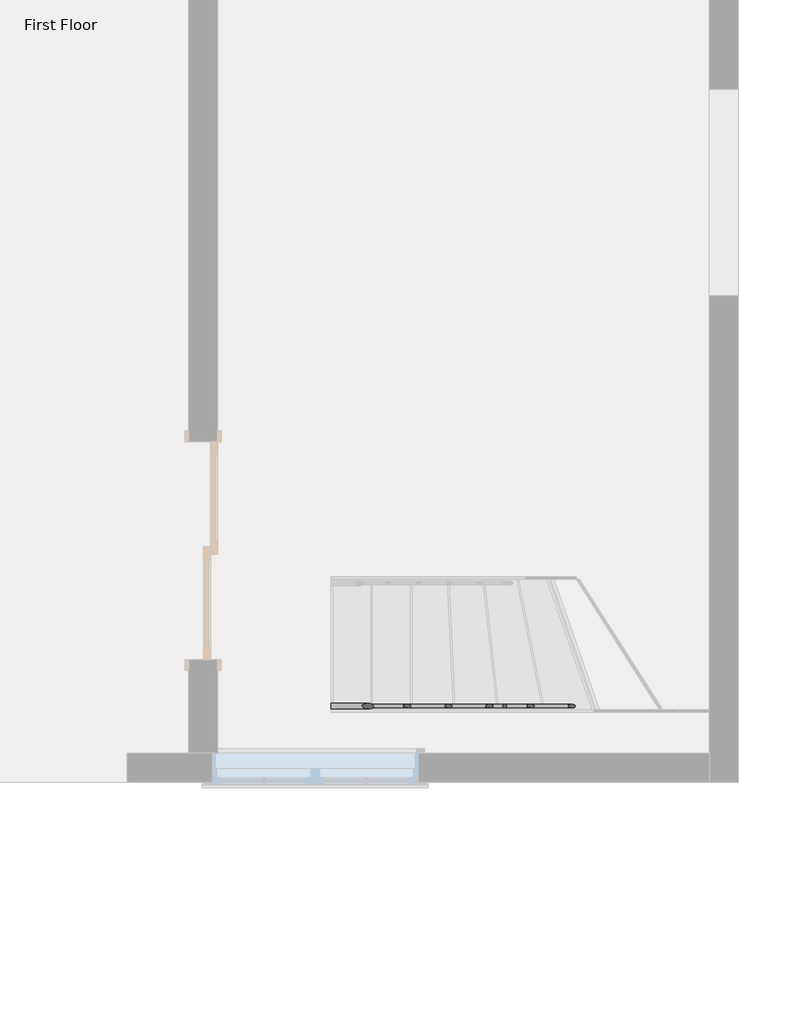
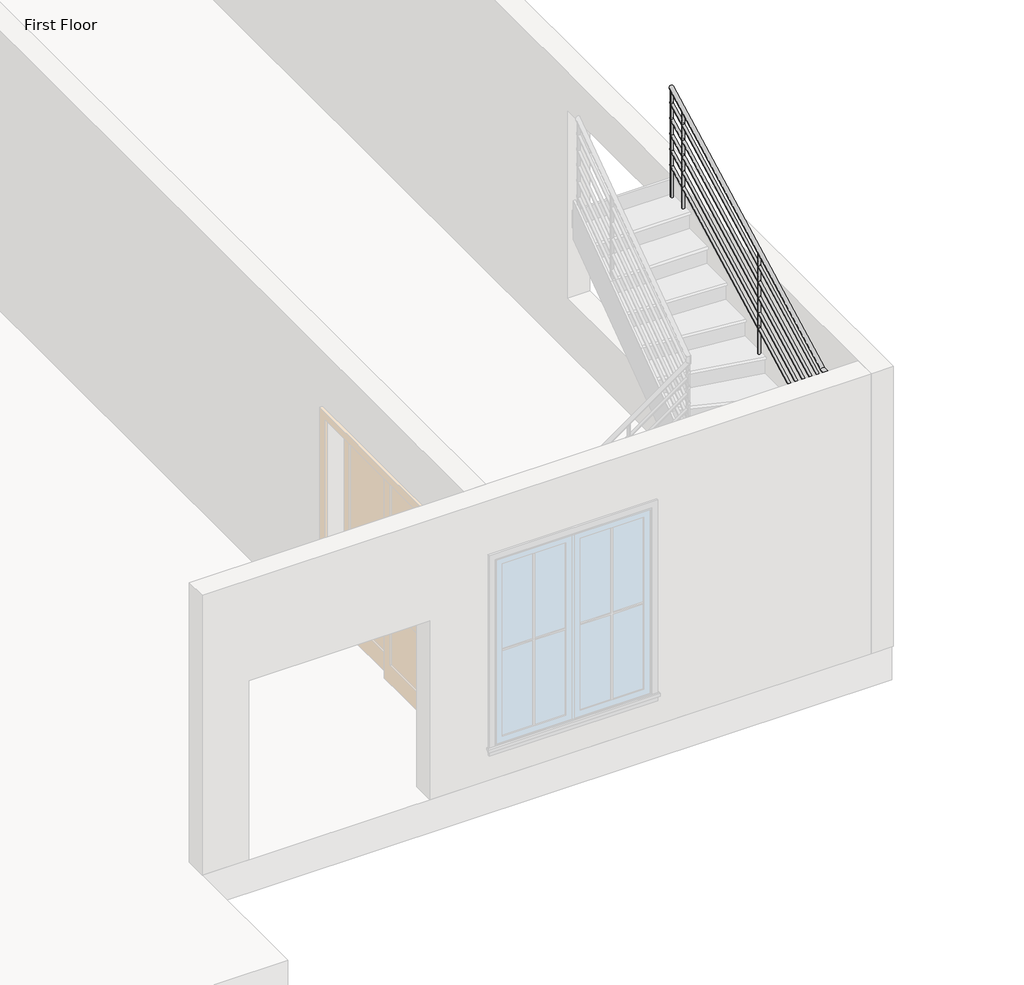
# One storey, part 3 of 4: 1 railing.
"""IFC4 building model written with IfcOpenShell, lengths in millimetres."""

from ifc_helpers import new_model, si_unit, point, frame, frame_2d, origin, place, context, project, spatial, circle_curve, ellipse_curve, trimmed, segment, composite_curve, outline, extrude, element, save
from ifc_brep_helpers import plane_surface, cylinder_surface, advanced_brep

model = new_model("IFC4")

# Units and contexts
model_context = context("Model", 3, world=origin())
ifc_project = project(units=[si_unit("LENGTHUNIT", "METRE", prefix="MILLI")], contexts=[model_context])

# Site, building, storey
site = spatial("IfcSite", under=ifc_project)
building = spatial("IfcBuilding", under=site)
storey = spatial("IfcBuildingStorey", under=building, Name="First Floor", Elevation=0.0)

# Railing
placement = place(None, origin())
element("IfcRailing", 1, ObjectType="Handrail - Pipe", at=placement, inside=storey, context=model_context, shape_type="SolidModel", body=[
    advanced_brep(
    [(6778.2616192, -13382.7029211, 1064.3134281), (6778.2616192, -13344.6029211, 1064.3134281), (9221.3605111, -13382.7029211, 2352.675), (9221.3605111, -13344.6029211, 2352.675), (9390.3486087, -13344.6029211, 2352.675), (9428.4486087, -13382.7029211, 2352.675), (9428.4486087, -13166.1843326, 2352.675), (9390.3486087, -13166.1843326, 2352.675), (9428.4486087, -10732.5159316, 3636.0634281), (9390.3486087, -10732.5159316, 3636.0634281)],
    [
        (0, 1, ellipse_curve(frame((6778.2616192, -13363.6529211, 1064.3134281), z_axis=(-1.0, 0.0, 0.0), x_axis=(0.0, 0.0, -1.0)), 21.5365719, 19.05)),
        (1, 0, ellipse_curve(frame((6778.2616192, -13363.6529211, 1064.3134281), z_axis=(-1.0, 0.0, 0.0), x_axis=(0.0, 0.0, -1.0)), 21.5365719, 19.05)),
        (0, 2),
        (2, 3, ellipse_curve(frame((9221.3605111, -13363.6529211, 2352.675), z_axis=(-0.9707064153254982, 0.0, -0.24026871466323146), x_axis=(0.2402687146632313, 0.0, -0.9707064153254984)), 19.6248832, 19.05)),
        (3, 1),
        (3, 2, ellipse_curve(frame((9221.3605111, -13363.6529211, 2352.675), z_axis=(-0.9707064153254982, 0.0, -0.24026871466323146), x_axis=(0.2402687146632313, 0.0, -0.9707064153254984)), 19.6248832, 19.05)),
        (4, 5, ellipse_curve(frame((9409.3986087, -13363.6529211, 2352.675), z_axis=(0.7071067811865475, 0.7071067811865475, 0.0), x_axis=(0.7071067811865474, -0.7071067811865476, 0.0)), 26.9407684, 19.05)),
        (5, 6),
        (6, 7, ellipse_curve(frame((9409.3986087, -13166.1843326, 2352.675), z_axis=(0.0, -0.9707064153254983, -0.2402687146632317), x_axis=(0.0, -0.24026871466323058, 0.9707064153254984)), 19.6248832, 19.05)),
        (7, 4),
        (5, 4, ellipse_curve(frame((9409.3986087, -13363.6529211, 2352.675), z_axis=(0.7071067811865475, 0.7071067811865475, 0.0), x_axis=(0.7071067811865474, -0.7071067811865476, 0.0)), 26.9407684, 19.05)),
        (7, 6, ellipse_curve(frame((9409.3986087, -13166.1843326, 2352.675), z_axis=(0.0, -0.9707064153254983, -0.2402687146632317), x_axis=(0.0, -0.24026871466323058, 0.9707064153254984)), 19.6248832, 19.05)),
        (2, 5),
        (4, 3),
        (8, 9, ellipse_curve(frame((9409.3986087, -10732.5159316, 3636.0634281), z_axis=(0.0, 1.0, 0.0), x_axis=(0.0, 0.0, -1.0)), 21.5365719, 19.05)),
        (9, 8, ellipse_curve(frame((9409.3986087, -10732.5159316, 3636.0634281), z_axis=(0.0, 1.0, 0.0), x_axis=(0.0, 0.0, -1.0)), 21.5365719, 19.05)),
        (6, 8),
        (9, 7),
    ],
    [
        plane_surface(frame((6778.2616192, -13363.6529211, 1085.85), z_axis=(-1.0, 0.0, 0.0), x_axis=(0.0, 1.0, 0.0))),
        cylinder_surface(frame((6787.1476968, -13363.6529211, 1068.999477), z_axis=(-0.8845418895081573, 0.0, -0.4664607654512208), x_axis=(0.0, 1.0, 0.0)), 19.05),
        cylinder_surface(frame((9409.3986087, -13363.6529211, 2352.675), z_axis=(0.0, -1.0, 0.0), x_axis=(-1.0, 0.0, 0.0)), 19.05),
        cylinder_surface(frame((9216.6452657, -13363.6529211, 2352.675), z_axis=(-1.0, 0.0, 0.0), x_axis=(0.0, 1.0, 0.0)), 19.05),
        plane_surface(frame((9409.3986087, -10732.5159316, 3657.6), z_axis=(0.0, 1.0, 0.0), x_axis=(0.0, 0.0, 1.0))),
        cylinder_surface(frame((9409.3986087, -13162.0135005, 2354.874477), z_axis=(0.0, -0.8845418895081572, -0.4664607654512212), x_axis=(-1.0, 0.0, 0.0)), 19.05),
    ],
    [
        (0, [[1, 2]]),
        (1, [[-1, 3, 4, 5]]),
        (1, [[-2, -5, 6, -3]]),
        (2, [[7, 8, 9, 10]]),
        (2, [[11, -10, 12, -8]]),
        (3, [[-4, 13, -7, 14]]),
        (3, [[-6, -14, -11, -13]]),
        (4, [[15, 16]]),
        (5, [[-9, 17, -16, 18]]),
        (5, [[-12, -18, -15, -17]]),
    ],
),
    advanced_brep(
    [(6778.2616192, -13350.9529211, 919.0922854), (6778.2616192, -13376.3529211, 919.0922854), (9219.7887626, -13350.9529211, 2206.625), (9219.7887626, -13376.3529211, 2206.625), (9396.6986087, -13350.9529211, 2206.625), (9396.6986087, -13376.3529211, 2206.625)],
    [
        (0, 1, ellipse_curve(frame((6778.2616192, -13363.6529211, 919.0922854), z_axis=(-1.0, 0.0, 0.0), x_axis=(0.0, 0.0, -1.0)), 14.3577146, 12.7)),
        (1, 0, ellipse_curve(frame((6778.2616192, -13363.6529211, 919.0922854), z_axis=(-1.0, 0.0, 0.0), x_axis=(0.0, 0.0, -1.0)), 14.3577146, 12.7)),
        (0, 2),
        (2, 3, ellipse_curve(frame((9219.7887626, -13363.6529211, 2206.625), z_axis=(-0.9707064153254982, 0.0, -0.24026871466323146), x_axis=(0.2402687146632313, 0.0, -0.9707064153254984)), 13.0832555, 12.7)),
        (3, 1),
        (3, 2, ellipse_curve(frame((9219.7887626, -13363.6529211, 2206.625), z_axis=(-0.9707064153254982, 0.0, -0.24026871466323146), x_axis=(0.2402687146632313, 0.0, -0.9707064153254984)), 13.0832555, 12.7)),
        (4, 5, circle_curve(frame((9396.6986087, -13363.6529211, 2206.625), z_axis=(1.0, 0.0, 0.0), x_axis=(0.0, -1.0, 0.0)), 12.7)),
        (5, 4, circle_curve(frame((9396.6986087, -13363.6529211, 2206.625), z_axis=(1.0, 0.0, 0.0), x_axis=(0.0, -1.0, 0.0)), 12.7)),
        (2, 4),
        (5, 3),
    ],
    [
        plane_surface(frame((6778.2616192, -13363.6529211, 933.45), z_axis=(-1.0, 0.0, 0.0), x_axis=(0.0, 1.0, 0.0))),
        cylinder_surface(frame((6784.185671, -13363.6529211, 922.216318), z_axis=(-0.8845418895081573, 0.0, -0.4664607654512208), x_axis=(0.0, -1.0, 0.0)), 12.7),
        plane_surface(frame((9396.6986087, -13363.6529211, 2219.325), z_axis=(1.0, 0.0, 0.0), x_axis=(0.0, 1.0, 0.0))),
        cylinder_surface(frame((9216.6452657, -13363.6529211, 2206.625), z_axis=(-1.0, 0.0, 0.0), x_axis=(0.0, -1.0, 0.0)), 12.7),
    ],
    [
        (0, [[1, 2]]),
        (1, [[-1, 3, 4, 5]]),
        (1, [[-2, -5, 6, -3]]),
        (2, [[7, 8]]),
        (3, [[-4, 9, -8, 10]]),
        (3, [[-6, -10, -7, -9]]),
    ],
),
    advanced_brep(
    [(9396.6986087, -13376.3529211, 2206.625), (9422.0986087, -13376.3529211, 2206.625), (9396.6986087, -13167.7560811, 2206.625), (9422.0986087, -13167.7560811, 2206.625), (9396.6986087, -10732.5159316, 3490.8422854), (9422.0986087, -10732.5159316, 3490.8422854)],
    [
        (0, 1, circle_curve(frame((9409.3986087, -13376.3529211, 2206.625), z_axis=(0.0, -1.0, 0.0), x_axis=(1.0, 0.0, 0.0)), 12.7)),
        (1, 0, circle_curve(frame((9409.3986087, -13376.3529211, 2206.625), z_axis=(0.0, -1.0, 0.0), x_axis=(1.0, 0.0, 0.0)), 12.7)),
        (0, 2),
        (2, 3, ellipse_curve(frame((9409.3986087, -13167.7560811, 2206.625), z_axis=(0.0, -0.9707064153254982, -0.24026871466323177), x_axis=(0.0, -0.2402687146632315, 0.9707064153254982)), 13.0832555, 12.7)),
        (3, 1),
        (3, 2, ellipse_curve(frame((9409.3986087, -13167.7560811, 2206.625), z_axis=(0.0, -0.9707064153254982, -0.24026871466323177), x_axis=(0.0, -0.2402687146632315, 0.9707064153254982)), 13.0832555, 12.7)),
        (4, 5, ellipse_curve(frame((9409.3986087, -10732.5159316, 3490.8422854), z_axis=(0.0, 1.0, 0.0), x_axis=(0.0, 0.0, -1.0)), 14.3577146, 12.7)),
        (5, 4, ellipse_curve(frame((9409.3986087, -10732.5159316, 3490.8422854), z_axis=(0.0, 1.0, 0.0), x_axis=(0.0, 0.0, -1.0)), 14.3577146, 12.7)),
        (2, 4),
        (5, 3),
    ],
    [
        plane_surface(frame((9409.3986087, -13376.3529211, 2219.325), z_axis=(0.0, -1.0, 0.0), x_axis=(0.0, 0.0, 1.0))),
        cylinder_surface(frame((9409.3986087, -13376.3529211, 2206.625), z_axis=(0.0, -1.0, 0.0), x_axis=(1.0, 0.0, 0.0)), 12.7),
        plane_surface(frame((9409.3986087, -10732.5159316, 3505.2), z_axis=(0.0, 1.0, 0.0), x_axis=(0.0, 0.0, 1.0))),
        cylinder_surface(frame((9409.3986087, -13164.9755263, 2208.091318), z_axis=(0.0, -0.884541889508157, -0.4664607654512213), x_axis=(1.0, 0.0, 0.0)), 12.7),
    ],
    [
        (0, [[1, 2]]),
        (1, [[-1, 3, 4, 5]]),
        (1, [[-2, -5, 6, -3]]),
        (2, [[7, 8]]),
        (3, [[-4, 9, -8, 10]]),
        (3, [[-6, -10, -7, -9]]),
    ],
),
    advanced_brep(
    [(6778.2616192, -13350.9529211, 766.6922854), (6778.2616192, -13376.3529211, 766.6922854), (9219.7887626, -13350.9529211, 2054.225), (9219.7887626, -13376.3529211, 2054.225), (9396.6986087, -13350.9529211, 2054.225), (9396.6986087, -13376.3529211, 2054.225)],
    [
        (0, 1, ellipse_curve(frame((6778.2616192, -13363.6529211, 766.6922854), z_axis=(-1.0, 0.0, 0.0), x_axis=(0.0, 0.0, -1.0)), 14.3577146, 12.7)),
        (1, 0, ellipse_curve(frame((6778.2616192, -13363.6529211, 766.6922854), z_axis=(-1.0, 0.0, 0.0), x_axis=(0.0, 0.0, -1.0)), 14.3577146, 12.7)),
        (0, 2),
        (2, 3, ellipse_curve(frame((9219.7887626, -13363.6529211, 2054.225), z_axis=(-0.9707064153254982, 0.0, -0.24026871466323146), x_axis=(0.2402687146632313, 0.0, -0.9707064153254984)), 13.0832555, 12.7)),
        (3, 1),
        (3, 2, ellipse_curve(frame((9219.7887626, -13363.6529211, 2054.225), z_axis=(-0.9707064153254982, 0.0, -0.24026871466323146), x_axis=(0.2402687146632313, 0.0, -0.9707064153254984)), 13.0832555, 12.7)),
        (4, 5, circle_curve(frame((9396.6986087, -13363.6529211, 2054.225), z_axis=(1.0, 0.0, 0.0), x_axis=(0.0, -1.0, 0.0)), 12.7)),
        (5, 4, circle_curve(frame((9396.6986087, -13363.6529211, 2054.225), z_axis=(1.0, 0.0, 0.0), x_axis=(0.0, -1.0, 0.0)), 12.7)),
        (2, 4),
        (5, 3),
    ],
    [
        plane_surface(frame((6778.2616192, -13363.6529211, 781.05), z_axis=(-1.0, 0.0, 0.0), x_axis=(0.0, 1.0, 0.0))),
        cylinder_surface(frame((6784.185671, -13363.6529211, 769.816318), z_axis=(-0.8845418895081573, 0.0, -0.4664607654512208), x_axis=(0.0, -1.0, 0.0)), 12.7),
        plane_surface(frame((9396.6986087, -13363.6529211, 2066.925), z_axis=(1.0, 0.0, 0.0), x_axis=(0.0, 1.0, 0.0))),
        cylinder_surface(frame((9216.6452657, -13363.6529211, 2054.225), z_axis=(-1.0, 0.0, 0.0), x_axis=(0.0, -1.0, 0.0)), 12.7),
    ],
    [
        (0, [[1, 2]]),
        (1, [[-1, 3, 4, 5]]),
        (1, [[-2, -5, 6, -3]]),
        (2, [[7, 8]]),
        (3, [[-4, 9, -8, 10]]),
        (3, [[-6, -10, -7, -9]]),
    ],
),
    advanced_brep(
    [(9396.6986087, -13376.3529211, 2054.225), (9422.0986087, -13376.3529211, 2054.225), (9396.6986087, -13167.7560811, 2054.225), (9422.0986087, -13167.7560811, 2054.225), (9396.6986087, -10732.5159316, 3338.4422854), (9422.0986087, -10732.5159316, 3338.4422854)],
    [
        (0, 1, circle_curve(frame((9409.3986087, -13376.3529211, 2054.225), z_axis=(0.0, -1.0, 0.0), x_axis=(1.0, 0.0, 0.0)), 12.7)),
        (1, 0, circle_curve(frame((9409.3986087, -13376.3529211, 2054.225), z_axis=(0.0, -1.0, 0.0), x_axis=(1.0, 0.0, 0.0)), 12.7)),
        (0, 2),
        (2, 3, ellipse_curve(frame((9409.3986087, -13167.7560811, 2054.225), z_axis=(0.0, -0.9707064153254982, -0.24026871466323177), x_axis=(0.0, -0.2402687146632315, 0.9707064153254982)), 13.0832555, 12.7)),
        (3, 1),
        (3, 2, ellipse_curve(frame((9409.3986087, -13167.7560811, 2054.225), z_axis=(0.0, -0.9707064153254982, -0.24026871466323177), x_axis=(0.0, -0.2402687146632315, 0.9707064153254982)), 13.0832555, 12.7)),
        (4, 5, ellipse_curve(frame((9409.3986087, -10732.5159316, 3338.4422854), z_axis=(0.0, 1.0, 0.0), x_axis=(0.0, 0.0, -1.0)), 14.3577146, 12.7)),
        (5, 4, ellipse_curve(frame((9409.3986087, -10732.5159316, 3338.4422854), z_axis=(0.0, 1.0, 0.0), x_axis=(0.0, 0.0, -1.0)), 14.3577146, 12.7)),
        (2, 4),
        (5, 3),
    ],
    [
        plane_surface(frame((9409.3986087, -13376.3529211, 2066.925), z_axis=(0.0, -1.0, 0.0), x_axis=(0.0, 0.0, 1.0))),
        cylinder_surface(frame((9409.3986087, -13376.3529211, 2054.225), z_axis=(0.0, -1.0, 0.0), x_axis=(1.0, 0.0, 0.0)), 12.7),
        plane_surface(frame((9409.3986087, -10732.5159316, 3352.8), z_axis=(0.0, 1.0, 0.0), x_axis=(0.0, 0.0, 1.0))),
        cylinder_surface(frame((9409.3986087, -13164.9755263, 2055.691318), z_axis=(0.0, -0.884541889508157, -0.4664607654512213), x_axis=(1.0, 0.0, 0.0)), 12.7),
    ],
    [
        (0, [[1, 2]]),
        (1, [[-1, 3, 4, 5]]),
        (1, [[-2, -5, 6, -3]]),
        (2, [[7, 8]]),
        (3, [[-4, 9, -8, 10]]),
        (3, [[-6, -10, -7, -9]]),
    ],
),
    advanced_brep(
    [(6778.2616192, -13350.9529211, 614.2922854), (6778.2616192, -13376.3529211, 614.2922854), (9219.7887626, -13350.9529211, 1901.825), (9219.7887626, -13376.3529211, 1901.825), (9396.6986087, -13350.9529211, 1901.825), (9396.6986087, -13376.3529211, 1901.825)],
    [
        (0, 1, ellipse_curve(frame((6778.2616192, -13363.6529211, 614.2922854), z_axis=(-1.0, 0.0, 0.0), x_axis=(0.0, 0.0, -1.0)), 14.3577146, 12.7)),
        (1, 0, ellipse_curve(frame((6778.2616192, -13363.6529211, 614.2922854), z_axis=(-1.0, 0.0, 0.0), x_axis=(0.0, 0.0, -1.0)), 14.3577146, 12.7)),
        (0, 2),
        (2, 3, ellipse_curve(frame((9219.7887626, -13363.6529211, 1901.825), z_axis=(-0.9707064153254982, 0.0, -0.24026871466323146), x_axis=(0.2402687146632313, 0.0, -0.9707064153254984)), 13.0832555, 12.7)),
        (3, 1),
        (3, 2, ellipse_curve(frame((9219.7887626, -13363.6529211, 1901.825), z_axis=(-0.9707064153254982, 0.0, -0.24026871466323146), x_axis=(0.2402687146632313, 0.0, -0.9707064153254984)), 13.0832555, 12.7)),
        (4, 5, circle_curve(frame((9396.6986087, -13363.6529211, 1901.825), z_axis=(1.0, 0.0, 0.0), x_axis=(0.0, -1.0, 0.0)), 12.7)),
        (5, 4, circle_curve(frame((9396.6986087, -13363.6529211, 1901.825), z_axis=(1.0, 0.0, 0.0), x_axis=(0.0, -1.0, 0.0)), 12.7)),
        (2, 4),
        (5, 3),
    ],
    [
        plane_surface(frame((6778.2616192, -13363.6529211, 628.65), z_axis=(-1.0, 0.0, 0.0), x_axis=(0.0, 1.0, 0.0))),
        cylinder_surface(frame((6784.185671, -13363.6529211, 617.416318), z_axis=(-0.8845418895081573, 0.0, -0.4664607654512208), x_axis=(0.0, -1.0, 0.0)), 12.7),
        plane_surface(frame((9396.6986087, -13363.6529211, 1914.525), z_axis=(1.0, 0.0, 0.0), x_axis=(0.0, 1.0, 0.0))),
        cylinder_surface(frame((9216.6452657, -13363.6529211, 1901.825), z_axis=(-1.0, 0.0, 0.0), x_axis=(0.0, -1.0, 0.0)), 12.7),
    ],
    [
        (0, [[1, 2]]),
        (1, [[-1, 3, 4, 5]]),
        (1, [[-2, -5, 6, -3]]),
        (2, [[7, 8]]),
        (3, [[-4, 9, -8, 10]]),
        (3, [[-6, -10, -7, -9]]),
    ],
),
    advanced_brep(
    [(9396.6986087, -13376.3529211, 1901.825), (9422.0986087, -13376.3529211, 1901.825), (9396.6986087, -13167.7560811, 1901.825), (9422.0986087, -13167.7560811, 1901.825), (9396.6986087, -10732.5159316, 3186.0422854), (9422.0986087, -10732.5159316, 3186.0422854)],
    [
        (0, 1, circle_curve(frame((9409.3986087, -13376.3529211, 1901.825), z_axis=(0.0, -1.0, 0.0), x_axis=(1.0, 0.0, 0.0)), 12.7)),
        (1, 0, circle_curve(frame((9409.3986087, -13376.3529211, 1901.825), z_axis=(0.0, -1.0, 0.0), x_axis=(1.0, 0.0, 0.0)), 12.7)),
        (0, 2),
        (2, 3, ellipse_curve(frame((9409.3986087, -13167.7560811, 1901.825), z_axis=(0.0, -0.9707064153254982, -0.24026871466323177), x_axis=(0.0, -0.2402687146632315, 0.9707064153254982)), 13.0832555, 12.7)),
        (3, 1),
        (3, 2, ellipse_curve(frame((9409.3986087, -13167.7560811, 1901.825), z_axis=(0.0, -0.9707064153254982, -0.24026871466323177), x_axis=(0.0, -0.2402687146632315, 0.9707064153254982)), 13.0832555, 12.7)),
        (4, 5, ellipse_curve(frame((9409.3986087, -10732.5159316, 3186.0422854), z_axis=(0.0, 1.0, 0.0), x_axis=(0.0, 0.0, -1.0)), 14.3577146, 12.7)),
        (5, 4, ellipse_curve(frame((9409.3986087, -10732.5159316, 3186.0422854), z_axis=(0.0, 1.0, 0.0), x_axis=(0.0, 0.0, -1.0)), 14.3577146, 12.7)),
        (2, 4),
        (5, 3),
    ],
    [
        plane_surface(frame((9409.3986087, -13376.3529211, 1914.525), z_axis=(0.0, -1.0, 0.0), x_axis=(0.0, 0.0, 1.0))),
        cylinder_surface(frame((9409.3986087, -13376.3529211, 1901.825), z_axis=(0.0, -1.0, 0.0), x_axis=(1.0, 0.0, 0.0)), 12.7),
        plane_surface(frame((9409.3986087, -10732.5159316, 3200.4), z_axis=(0.0, 1.0, 0.0), x_axis=(0.0, 0.0, 1.0))),
        cylinder_surface(frame((9409.3986087, -13164.9755263, 1903.291318), z_axis=(0.0, -0.884541889508157, -0.4664607654512213), x_axis=(1.0, 0.0, 0.0)), 12.7),
    ],
    [
        (0, [[1, 2]]),
        (1, [[-1, 3, 4, 5]]),
        (1, [[-2, -5, 6, -3]]),
        (2, [[7, 8]]),
        (3, [[-4, 9, -8, 10]]),
        (3, [[-6, -10, -7, -9]]),
    ],
),
    advanced_brep(
    [(6778.2616192, -13350.9529211, 461.8922854), (6778.2616192, -13376.3529211, 461.8922854), (9219.7887626, -13350.9529211, 1749.425), (9219.7887626, -13376.3529211, 1749.425), (9396.6986087, -13350.9529211, 1749.425), (9396.6986087, -13376.3529211, 1749.425)],
    [
        (0, 1, ellipse_curve(frame((6778.2616192, -13363.6529211, 461.8922854), z_axis=(-1.0, 0.0, 0.0), x_axis=(0.0, 0.0, -1.0)), 14.3577146, 12.7)),
        (1, 0, ellipse_curve(frame((6778.2616192, -13363.6529211, 461.8922854), z_axis=(-1.0, 0.0, 0.0), x_axis=(0.0, 0.0, -1.0)), 14.3577146, 12.7)),
        (0, 2),
        (2, 3, ellipse_curve(frame((9219.7887626, -13363.6529211, 1749.425), z_axis=(-0.9707064153254982, 0.0, -0.24026871466323146), x_axis=(0.2402687146632313, 0.0, -0.9707064153254984)), 13.0832555, 12.7)),
        (3, 1),
        (3, 2, ellipse_curve(frame((9219.7887626, -13363.6529211, 1749.425), z_axis=(-0.9707064153254982, 0.0, -0.24026871466323146), x_axis=(0.2402687146632313, 0.0, -0.9707064153254984)), 13.0832555, 12.7)),
        (4, 5, circle_curve(frame((9396.6986087, -13363.6529211, 1749.425), z_axis=(1.0, 0.0, 0.0), x_axis=(0.0, -1.0, 0.0)), 12.7)),
        (5, 4, circle_curve(frame((9396.6986087, -13363.6529211, 1749.425), z_axis=(1.0, 0.0, 0.0), x_axis=(0.0, -1.0, 0.0)), 12.7)),
        (2, 4),
        (5, 3),
    ],
    [
        plane_surface(frame((6778.2616192, -13363.6529211, 476.25), z_axis=(-1.0, 0.0, 0.0), x_axis=(0.0, 1.0, 0.0))),
        cylinder_surface(frame((6784.185671, -13363.6529211, 465.016318), z_axis=(-0.8845418895081573, 0.0, -0.4664607654512208), x_axis=(0.0, -1.0, 0.0)), 12.7),
        plane_surface(frame((9396.6986087, -13363.6529211, 1762.125), z_axis=(1.0, 0.0, 0.0), x_axis=(0.0, 1.0, 0.0))),
        cylinder_surface(frame((9216.6452657, -13363.6529211, 1749.425), z_axis=(-1.0, 0.0, 0.0), x_axis=(0.0, -1.0, 0.0)), 12.7),
    ],
    [
        (0, [[1, 2]]),
        (1, [[-1, 3, 4, 5]]),
        (1, [[-2, -5, 6, -3]]),
        (2, [[7, 8]]),
        (3, [[-4, 9, -8, 10]]),
        (3, [[-6, -10, -7, -9]]),
    ],
),
    advanced_brep(
    [(9396.6986087, -13376.3529211, 1749.425), (9422.0986087, -13376.3529211, 1749.425), (9396.6986087, -13167.7560811, 1749.425), (9422.0986087, -13167.7560811, 1749.425), (9396.6986087, -10732.5159316, 3033.6422854), (9422.0986087, -10732.5159316, 3033.6422854)],
    [
        (0, 1, circle_curve(frame((9409.3986087, -13376.3529211, 1749.425), z_axis=(0.0, -1.0, 0.0), x_axis=(1.0, 0.0, 0.0)), 12.7)),
        (1, 0, circle_curve(frame((9409.3986087, -13376.3529211, 1749.425), z_axis=(0.0, -1.0, 0.0), x_axis=(1.0, 0.0, 0.0)), 12.7)),
        (0, 2),
        (2, 3, ellipse_curve(frame((9409.3986087, -13167.7560811, 1749.425), z_axis=(0.0, -0.9707064153254982, -0.24026871466323177), x_axis=(0.0, -0.2402687146632315, 0.9707064153254982)), 13.0832555, 12.7)),
        (3, 1),
        (3, 2, ellipse_curve(frame((9409.3986087, -13167.7560811, 1749.425), z_axis=(0.0, -0.9707064153254982, -0.24026871466323177), x_axis=(0.0, -0.2402687146632315, 0.9707064153254982)), 13.0832555, 12.7)),
        (4, 5, ellipse_curve(frame((9409.3986087, -10732.5159316, 3033.6422854), z_axis=(0.0, 1.0, 0.0), x_axis=(0.0, 0.0, -1.0)), 14.3577146, 12.7)),
        (5, 4, ellipse_curve(frame((9409.3986087, -10732.5159316, 3033.6422854), z_axis=(0.0, 1.0, 0.0), x_axis=(0.0, 0.0, -1.0)), 14.3577146, 12.7)),
        (2, 4),
        (5, 3),
    ],
    [
        plane_surface(frame((9409.3986087, -13376.3529211, 1762.125), z_axis=(0.0, -1.0, 0.0), x_axis=(0.0, 0.0, 1.0))),
        cylinder_surface(frame((9409.3986087, -13376.3529211, 1749.425), z_axis=(0.0, -1.0, 0.0), x_axis=(1.0, 0.0, 0.0)), 12.7),
        plane_surface(frame((9409.3986087, -10732.5159316, 3048.0), z_axis=(0.0, 1.0, 0.0), x_axis=(0.0, 0.0, 1.0))),
        cylinder_surface(frame((9409.3986087, -13164.9755263, 1750.891318), z_axis=(0.0, -0.884541889508157, -0.4664607654512213), x_axis=(1.0, 0.0, 0.0)), 12.7),
    ],
    [
        (0, [[1, 2]]),
        (1, [[-1, 3, 4, 5]]),
        (1, [[-2, -5, 6, -3]]),
        (2, [[7, 8]]),
        (3, [[-4, 9, -8, 10]]),
        (3, [[-6, -10, -7, -9]]),
    ],
),
    advanced_brep(
    [(6778.2616192, -13350.9529211, 309.4922854), (6778.2616192, -13376.3529211, 309.4922854), (9219.7887626, -13350.9529211, 1597.025), (9219.7887626, -13376.3529211, 1597.025), (9396.6986087, -13350.9529211, 1597.025), (9396.6986087, -13376.3529211, 1597.025)],
    [
        (0, 1, ellipse_curve(frame((6778.2616192, -13363.6529211, 309.4922854), z_axis=(-1.0, 0.0, 0.0), x_axis=(0.0, 0.0, -1.0)), 14.3577146, 12.7)),
        (1, 0, ellipse_curve(frame((6778.2616192, -13363.6529211, 309.4922854), z_axis=(-1.0, 0.0, 0.0), x_axis=(0.0, 0.0, -1.0)), 14.3577146, 12.7)),
        (0, 2),
        (2, 3, ellipse_curve(frame((9219.7887626, -13363.6529211, 1597.025), z_axis=(-0.9707064153254982, 0.0, -0.24026871466323146), x_axis=(0.2402687146632313, 0.0, -0.9707064153254984)), 13.0832555, 12.7)),
        (3, 1),
        (3, 2, ellipse_curve(frame((9219.7887626, -13363.6529211, 1597.025), z_axis=(-0.9707064153254982, 0.0, -0.24026871466323146), x_axis=(0.2402687146632313, 0.0, -0.9707064153254984)), 13.0832555, 12.7)),
        (4, 5, circle_curve(frame((9396.6986087, -13363.6529211, 1597.025), z_axis=(1.0, 0.0, 0.0), x_axis=(0.0, -1.0, 0.0)), 12.7)),
        (5, 4, circle_curve(frame((9396.6986087, -13363.6529211, 1597.025), z_axis=(1.0, 0.0, 0.0), x_axis=(0.0, -1.0, 0.0)), 12.7)),
        (2, 4),
        (5, 3),
    ],
    [
        plane_surface(frame((6778.2616192, -13363.6529211, 323.85), z_axis=(-1.0, 0.0, 0.0), x_axis=(0.0, 1.0, 0.0))),
        cylinder_surface(frame((6784.185671, -13363.6529211, 312.616318), z_axis=(-0.8845418895081573, 0.0, -0.4664607654512208), x_axis=(0.0, -1.0, 0.0)), 12.7),
        plane_surface(frame((9396.6986087, -13363.6529211, 1609.725), z_axis=(1.0, 0.0, 0.0), x_axis=(0.0, 1.0, 0.0))),
        cylinder_surface(frame((9216.6452657, -13363.6529211, 1597.025), z_axis=(-1.0, 0.0, 0.0), x_axis=(0.0, -1.0, 0.0)), 12.7),
    ],
    [
        (0, [[1, 2]]),
        (1, [[-1, 3, 4, 5]]),
        (1, [[-2, -5, 6, -3]]),
        (2, [[7, 8]]),
        (3, [[-4, 9, -8, 10]]),
        (3, [[-6, -10, -7, -9]]),
    ],
),
    advanced_brep(
    [(9396.6986087, -13376.3529211, 1597.025), (9422.0986087, -13376.3529211, 1597.025), (9396.6986087, -13167.7560811, 1597.025), (9422.0986087, -13167.7560811, 1597.025), (9396.6986087, -10732.5159316, 2881.2422854), (9422.0986087, -10732.5159316, 2881.2422854)],
    [
        (0, 1, circle_curve(frame((9409.3986087, -13376.3529211, 1597.025), z_axis=(0.0, -1.0, 0.0), x_axis=(1.0, 0.0, 0.0)), 12.7)),
        (1, 0, circle_curve(frame((9409.3986087, -13376.3529211, 1597.025), z_axis=(0.0, -1.0, 0.0), x_axis=(1.0, 0.0, 0.0)), 12.7)),
        (0, 2),
        (2, 3, ellipse_curve(frame((9409.3986087, -13167.7560811, 1597.025), z_axis=(0.0, -0.9707064153254982, -0.24026871466323177), x_axis=(0.0, -0.2402687146632315, 0.9707064153254982)), 13.0832555, 12.7)),
        (3, 1),
        (3, 2, ellipse_curve(frame((9409.3986087, -13167.7560811, 1597.025), z_axis=(0.0, -0.9707064153254982, -0.24026871466323177), x_axis=(0.0, -0.2402687146632315, 0.9707064153254982)), 13.0832555, 12.7)),
        (4, 5, ellipse_curve(frame((9409.3986087, -10732.5159316, 2881.2422854), z_axis=(0.0, 1.0, 0.0), x_axis=(0.0, 0.0, -1.0)), 14.3577146, 12.7)),
        (5, 4, ellipse_curve(frame((9409.3986087, -10732.5159316, 2881.2422854), z_axis=(0.0, 1.0, 0.0), x_axis=(0.0, 0.0, -1.0)), 14.3577146, 12.7)),
        (2, 4),
        (5, 3),
    ],
    [
        plane_surface(frame((9409.3986087, -13376.3529211, 1609.725), z_axis=(0.0, -1.0, 0.0), x_axis=(0.0, 0.0, 1.0))),
        cylinder_surface(frame((9409.3986087, -13376.3529211, 1597.025), z_axis=(0.0, -1.0, 0.0), x_axis=(1.0, 0.0, 0.0)), 12.7),
        plane_surface(frame((9409.3986087, -10732.5159316, 2895.6), z_axis=(0.0, 1.0, 0.0), x_axis=(0.0, 0.0, 1.0))),
        cylinder_surface(frame((9409.3986087, -13164.9755263, 1598.491318), z_axis=(0.0, -0.884541889508157, -0.4664607654512213), x_axis=(1.0, 0.0, 0.0)), 12.7),
    ],
    [
        (0, [[1, 2]]),
        (1, [[-1, 3, 4, 5]]),
        (1, [[-2, -5, 6, -3]]),
        (2, [[7, 8]]),
        (3, [[-4, 9, -8, 10]]),
        (3, [[-6, -10, -7, -9]]),
    ],
),
    advanced_brep(
    [(9422.0986087, -10925.2529211, 3512.8875277), (9422.0986087, -10925.2529211, 2571.75), (9396.6986087, -10925.2529211, 2571.75), (9396.6986087, -10925.2529211, 3512.8875277)],
    [
        (0, 1),
        (1, 2, circle_curve(frame((9409.3986087, -10925.2529211, 2571.75), z_axis=(0.0, 0.0, 1.0), x_axis=(-1.0, 0.0, 0.0)), 12.7)),
        (2, 3),
        (3, 0, ellipse_curve(frame((9409.3986087, -10925.2529211, 3512.8875277), z_axis=(0.0, 0.4664607654512186, -0.8845418895081586), x_axis=(0.0, 0.8845418895081587, 0.4664607654512182)), 14.3577146, 12.7)),
        (0, 3, ellipse_curve(frame((9409.3986087, -10925.2529211, 3512.8875277), z_axis=(0.0, 0.4664607654512186, -0.8845418895081586), x_axis=(0.0, 0.8845418895081587, 0.4664607654512182)), 14.3577146, 12.7)),
        (2, 1, circle_curve(frame((9409.3986087, -10925.2529211, 2571.75), z_axis=(0.0, 0.0, 1.0), x_axis=(-1.0, 0.0, 0.0)), 12.7)),
    ],
    [
        cylinder_surface(frame((9409.3986087, -10925.2529211, 2343.15), z_axis=(0.0, 0.0, 1.0), x_axis=(-1.0, 0.0, 0.0)), 12.7),
        plane_surface(frame((9383.9986087, -10899.8529211, 3526.2821488), z_axis=(0.0, -0.4664607654512186, 0.8845418895081586), x_axis=(1.0, 0.0, 0.0))),
        plane_surface(frame((9383.9986087, -10950.6529211, 2571.75), z_axis=(0.0, 0.0, -1.0), x_axis=(1.0, 0.0, 0.0))),
    ],
    [
        (0, [[1, 2, 3, 4]]),
        (0, [[-1, 5, -3, 6]]),
        (1, [[-4, -5]]),
        (2, [[-2, -6]]),
    ],
),
    advanced_brep(
    [(9422.0986087, -12144.4529211, 2869.9457157), (9422.0986087, -12144.4529211, 1885.95), (9396.6986087, -12144.4529211, 1885.95), (9396.6986087, -12144.4529211, 2869.9457157)],
    [
        (0, 1),
        (1, 2, circle_curve(frame((9409.3986087, -12144.4529211, 1885.95), z_axis=(0.0, 0.0, 1.0), x_axis=(-1.0, 0.0, 0.0)), 12.7)),
        (2, 3),
        (3, 0, ellipse_curve(frame((9409.3986087, -12144.4529211, 2869.9457157), z_axis=(0.0, 0.4664607654512186, -0.8845418895081586), x_axis=(0.0, 0.8845418895081587, 0.4664607654512182)), 14.3577146, 12.7)),
        (0, 3, ellipse_curve(frame((9409.3986087, -12144.4529211, 2869.9457157), z_axis=(0.0, 0.4664607654512186, -0.8845418895081586), x_axis=(0.0, 0.8845418895081587, 0.4664607654512182)), 14.3577146, 12.7)),
        (2, 1, circle_curve(frame((9409.3986087, -12144.4529211, 1885.95), z_axis=(0.0, 0.0, 1.0), x_axis=(-1.0, 0.0, 0.0)), 12.7)),
    ],
    [
        cylinder_surface(frame((9409.3986087, -12144.4529211, 1657.35), z_axis=(0.0, 0.0, 1.0), x_axis=(-1.0, 0.0, 0.0)), 12.7),
        plane_surface(frame((9383.9986087, -12119.0529211, 2883.3403368), z_axis=(0.0, -0.4664607654512186, 0.8845418895081586), x_axis=(1.0, 0.0, 0.0))),
        plane_surface(frame((9383.9986087, -12169.8529211, 1885.95), z_axis=(0.0, 0.0, -1.0), x_axis=(1.0, 0.0, 0.0))),
    ],
    [
        (0, [[1, 2, 3, 4]]),
        (0, [[-1, 5, -3, 6]]),
        (1, [[-4, -5]]),
        (2, [[-2, -6]]),
    ],
),
    extrude(outline(composite_curve([segment(trimmed(circle_curve(frame_2d((9216.6616192, -13363.6529211)), 12.7), [point((9216.6616192, -13350.9529211))], [point((9216.6616192, -13376.3529211))], False, "CARTESIAN"), True, "CONTINUOUS"), segment(trimmed(circle_curve(frame_2d((9216.6616192, -13363.6529211)), 12.7), [point((9216.6616192, -13376.3529211))], [point((9216.6616192, -13350.9529211))], False, "CARTESIAN"), True, "CONTINUOUS")], self_intersect=False)), frame((0.0, 0.0, 1371.6), z_axis=(0.0, 0.0, 1.0), x_axis=(1.0, 0.0, 0.0)), (0.0, 0.0, 1.0), 962.025),
    advanced_brep(
    [(7997.4616192, -13376.3529211, 1685.7186682), (7997.4616192, -13376.3529211, 857.25), (7997.4616192, -13350.9529211, 857.25), (7997.4616192, -13350.9529211, 1685.7186682)],
    [
        (0, 1),
        (1, 2, circle_curve(frame((7997.4616192, -13363.6529211, 857.25), z_axis=(0.0, 0.0, 1.0), x_axis=(0.0, 1.0, 0.0)), 12.7)),
        (2, 3),
        (3, 0, ellipse_curve(frame((7997.4616192, -13363.6529211, 1685.7186682), z_axis=(0.4664607654512186, 0.0, -0.8845418895081586), x_axis=(0.8845418895081587, 0.0, 0.4664607654512182)), 14.3577146, 12.7)),
        (0, 3, ellipse_curve(frame((7997.4616192, -13363.6529211, 1685.7186682), z_axis=(0.4664607654512186, 0.0, -0.8845418895081586), x_axis=(0.8845418895081587, 0.0, 0.4664607654512182)), 14.3577146, 12.7)),
        (2, 1, circle_curve(frame((7997.4616192, -13363.6529211, 857.25), z_axis=(0.0, 0.0, 1.0), x_axis=(0.0, 1.0, 0.0)), 12.7)),
    ],
    [
        cylinder_surface(frame((7997.4616192, -13363.6529211, 628.65), z_axis=(0.0, 0.0, 1.0), x_axis=(0.0, 1.0, 0.0)), 12.7),
        plane_surface(frame((8022.8616192, -13338.2529211, 1699.1132893), z_axis=(-0.4664607654512186, 0.0, 0.8845418895081586), x_axis=(0.0, -1.0, 0.0))),
        plane_surface(frame((7972.0616192, -13338.2529211, 857.25), z_axis=(0.0, 0.0, -1.0), x_axis=(0.0, -1.0, 0.0))),
    ],
    [
        (0, [[1, 2, 3, 4]]),
        (0, [[-1, 5, -3, 6]]),
        (1, [[-4, -5]]),
        (2, [[-2, -6]]),
    ],
),
    extrude(outline(composite_curve([segment(trimmed(circle_curve(frame_2d((9409.3986087, -13363.6529211)), 12.7), [point((9409.3986087, -13350.9529211))], [point((9409.3986087, -13376.3529211))], False, "CARTESIAN"), True, "CONTINUOUS"), segment(trimmed(circle_curve(frame_2d((9409.3986087, -13363.6529211)), 12.7), [point((9409.3986087, -13376.3529211))], [point((9409.3986087, -13350.9529211))], False, "CARTESIAN"), True, "CONTINUOUS")], self_intersect=False)), frame((0.0, 0.0, 1371.6), z_axis=(0.0, 0.0, 1.0), x_axis=(1.0, 0.0, 0.0)), (0.0, 0.0, 1.0), 962.025),
    advanced_brep(
    [(9422.0986087, -10745.2159316, 3607.8295457), (9422.0986087, -10745.2159316, 2571.75), (9396.6986087, -10745.2159316, 2571.75), (9396.6986087, -10745.2159316, 3607.8295457)],
    [
        (0, 1),
        (1, 2, circle_curve(frame((9409.3986087, -10745.2159316, 2571.75), z_axis=(0.0, 0.0, 1.0), x_axis=(-1.0, 0.0, 0.0)), 12.7)),
        (2, 3),
        (3, 0, ellipse_curve(frame((9409.3986087, -10745.2159316, 3607.8295457), z_axis=(0.0, 0.4664607654512186, -0.8845418895081586), x_axis=(0.0, 0.8845418895081587, 0.4664607654512182)), 14.3577146, 12.7)),
        (0, 3, ellipse_curve(frame((9409.3986087, -10745.2159316, 3607.8295457), z_axis=(0.0, 0.4664607654512186, -0.8845418895081586), x_axis=(0.0, 0.8845418895081587, 0.4664607654512182)), 14.3577146, 12.7)),
        (2, 1, circle_curve(frame((9409.3986087, -10745.2159316, 2571.75), z_axis=(0.0, 0.0, 1.0), x_axis=(-1.0, 0.0, 0.0)), 12.7)),
    ],
    [
        cylinder_surface(frame((9409.3986087, -10745.2159316, 2343.15), z_axis=(0.0, 0.0, 1.0), x_axis=(-1.0, 0.0, 0.0)), 12.7),
        plane_surface(frame((9383.9986087, -10719.8159316, 3621.2241667), z_axis=(0.0, -0.4664607654512186, 0.8845418895081586), x_axis=(1.0, 0.0, 0.0))),
        plane_surface(frame((9383.9986087, -10770.6159316, 2571.75), z_axis=(0.0, 0.0, -1.0), x_axis=(1.0, 0.0, 0.0))),
    ],
    [
        (0, [[1, 2, 3, 4]]),
        (0, [[-1, 5, -3, 6]]),
        (1, [[-4, -5]]),
        (2, [[-2, -6]]),
    ],
),
    advanced_brep(
    [(6790.9616192, -13376.3529211, 1049.4741667), (6790.9616192, -13376.3529211, 171.45), (6790.9616192, -13350.9529211, 171.45), (6790.9616192, -13350.9529211, 1049.4741667)],
    [
        (0, 1),
        (1, 2, circle_curve(frame((6790.9616192, -13363.6529211, 171.45), z_axis=(0.0, 0.0, 1.0), x_axis=(0.0, 1.0, 0.0)), 12.7)),
        (2, 3),
        (3, 0, ellipse_curve(frame((6790.9616192, -13363.6529211, 1049.4741667), z_axis=(0.46646076545122045, 0.0, -0.8845418895081575), x_axis=(0.8845418895081574, 0.0, 0.4664607654512205)), 14.3577146, 12.7)),
        (0, 3, ellipse_curve(frame((6790.9616192, -13363.6529211, 1049.4741667), z_axis=(0.46646076545122045, 0.0, -0.8845418895081575), x_axis=(0.8845418895081574, 0.0, 0.4664607654512205)), 14.3577146, 12.7)),
        (2, 1, circle_curve(frame((6790.9616192, -13363.6529211, 171.45), z_axis=(0.0, 0.0, 1.0), x_axis=(0.0, 1.0, 0.0)), 12.7)),
    ],
    [
        cylinder_surface(frame((6790.9616192, -13363.6529211, -57.15), z_axis=(0.0, 0.0, 1.0), x_axis=(0.0, 1.0, 0.0)), 12.7),
        plane_surface(frame((6816.3616192, -13338.2529211, 1062.8687878), z_axis=(-0.46646076545122045, 0.0, 0.8845418895081575), x_axis=(0.0, -1.0, 0.0))),
        plane_surface(frame((6765.5616192, -13338.2529211, 171.45), z_axis=(0.0, 0.0, -1.0), x_axis=(0.0, -1.0, 0.0))),
    ],
    [
        (0, [[1, 2, 3, 4]]),
        (0, [[-1, 5, -3, 6]]),
        (1, [[-4, -5]]),
        (2, [[-2, -6]]),
    ],
),
])

save(model, "model.ifc")

# Revit data of these elements
# Type "Handrail - Pipe"
#   Assembly Code = "C2010400"
#   built-in parameter 1008612 = 0.0416667 (stored number, unit not read)
#   built-in parameter 1008611 = 0.0833333 (stored number, unit not read)
#   built-in parameter 1008609 = 4 (stored number, unit not read)
#   built-in parameter 1008604 = 0.166667 (stored number, unit not read)
#   built-in parameter 1008603 = 0.166667 (stored number, unit not read)
#   Railing Height = 3' - 0"
#   built-in parameter 1008630 = 2
#   built-in parameter 1008610 = 1
#   built-in parameter 1008605 = 1
#   built-in parameter 1008618 = Baluster - Round : 1"
# Element 1 (IfcRailing, "Handrail - Pipe")
#   Phase Created = New Construction
# Room at (-618.762, -12798.192) mm, phase "New Construction", upper level "First Floor", upper offset 9' - 0", lower offset 0' - 0"
#   Number = "1"
#   Name = "Drawing Room"
# Room at (-1533.162, -7930.102) mm, phase "New Construction", upper level "First Floor", upper offset 9' - 0", lower offset 0' - 0"
#   Number = "2"
#   Name = "Parents Room"
# Room at (4087.125, -9236.455) mm, phase "New Construction", upper level "First Floor", upper offset 9' - 0", lower offset 0' - 0"
#   Number = "3"
#   Name = "Reception Hall"
# Room at (7364.078, -9635.003) mm, phase "New Construction", upper level "First Floor", upper offset 9' - 0", lower offset 0' - 0"
#   Number = "4"
#   Name = "Stair-Hall"
# Room at (7076.238, -3878.194) mm, phase "New Construction", upper level "First Floor", upper offset 9' - 0", lower offset 0' - 0"
#   Number = "5"
#   Name = "Kitchen-Main"
# Room at (1414.821, -2931.311) mm, phase "New Construction", upper level "First Floor", upper offset 9' - 0", lower offset 0' - 0"
#   Number = "6"
#   Name = "TV Room"
# Room at (6753.594, 2096.463) mm, phase "New Construction", upper level "First Floor", upper offset 9' - 0", lower offset 0' - 0"
#   Number = "7"
#   Name = "Bed-Ali"
# Room at (-179.257, 5421.57) mm, phase "New Construction", upper level "First Floor", upper offset 9' - 0", lower offset 0' - 0"
#   Number = "10"
#   Name = "Bath-Kazim"
# Room at (3517.157, 5421.57) mm, phase "New Construction", upper level "First Floor", upper offset 9' - 0", lower offset 0' - 0"
#   Number = "11"
#   Name = "Bed-Kazim"
# Room at (7076.238, -1361.648) mm, phase "New Construction", upper level "First Floor", upper offset 9' - 0", lower offset 0' - 0"
#   Number = "13"
#   Name = "Kitchen-dirty"
# Room at (-1093.657, 2096.463) mm, phase "New Construction", upper level "First Floor", upper offset 9' - 0", lower offset 0' - 0"
#   Number = "8"
#   Name = "Bed-Ahsin"
# Room at (-2447.562, 5421.57) mm, phase "New Construction", upper level "First Floor", upper offset 9' - 0", lower offset 0' - 0"
#   Number = "9"
#   Name = "Bath-Ahsin"
# Room at (8238.808, 5421.57) mm, phase "New Construction", upper level "First Floor", upper offset 9' - 0", lower offset 0' - 0"
#   Number = "12"
#   Name = "Bath-Ali"
